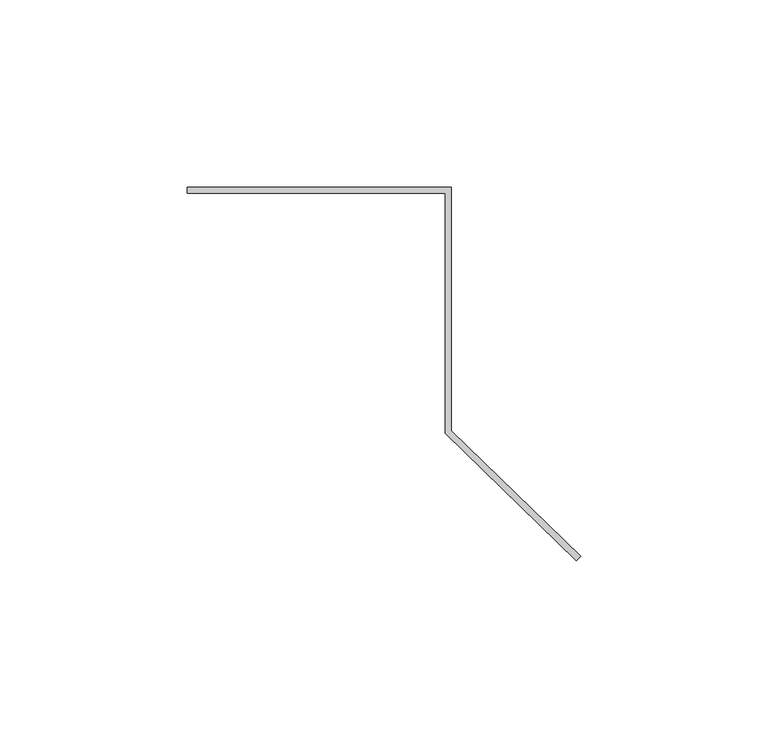
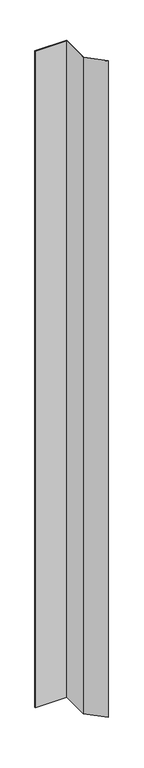
"""IFC4 building model written with IfcOpenShell, lengths in millimetres: proxy geometry, Generic Models 2:Generic Models 2:310765:Generic Models 2:310765 : Generic Models 2:Generic Models 2:310765:61 : Generic Models 2:Generic Models 2:310765:Generic Models 2:310765 : Generic Models 2:Generic Models 2:310765:300385."""

from ifc_helpers import new_model, si_unit, frame, origin, place, context, project, spatial, polyline, outline, extrude, source, transform, mapped, element, save


def generic_models_9b77d285(model_context):
    return source(origin(), model_context, "Body", "SweptSolid", [
        extrude(outline(polyline([(667216.6366489, -568274.0939933), (667286.9617239, -568274.0939933), (667286.9617239, -568339.0177162), (667321.5133229, -568372.5097328), (667320.3906548, -568373.6324009), (667285.3742239, -568339.6898072), (667285.3742239, -568275.6814933), (667216.6366489, -568275.6814933), (667216.6366489, -568274.0939933)])), frame((0.0, 0.0, 4636.9670756), z_axis=(0.0, 0.0, 1.0), x_axis=(1.0, 0.0, 0.0)), (0.0, 0.0, 1.0), 1528.8829244),
    ])


if __name__ == "__main__":
    model = new_model("IFC4")
    model_context = context("Model", 3, world=origin())
    ifc_project = project(units=[si_unit("LENGTHUNIT", "METRE", prefix="MILLI")], contexts=[model_context])
    site = spatial("IfcSite", under=ifc_project)
    building = spatial("IfcBuilding", under=site)
    placement = place(None, origin())
    generic_models_shape = generic_models_9b77d285(model_context)
    element("IfcBuildingElementProxy", 1, Name="Generic Models 2:Generic Models 2:310765:Generic Models 2:310765 : Generic Models 2:Generic Models 2:310765:61 : Generic Models 2:Generic Models 2:310765:Generic Models 2:310765 : Generic Models 2:Generic Models 2:310765:300385", ObjectType="Generic Models 2:Generic Models 2:310765:Generic Models 2:310765 : Generic Models 2:Generic Models 2:310765:61 : Generic Models 2:Generic Models 2:310765:Generic Models 2:310765 : Generic Models 2:Generic Models 2:310765:300385", at=placement, inside=building, context=model_context, shape_type="MappedRepresentation", body=[
        mapped(generic_models_shape, transform((0.0, 0.0, 0.0), x_axis=(1.0, 0.0, 0.0), y_axis=(0.0, 1.0, 0.0), z_axis=(0.0, 0.0, 1.0))),
    ])
    save(model, "model.ifc")

# Revit data of these elements
# Type "Generic Models 2:Generic Models 2:310765:Generic Models 2:310765 : Generic Models 2:Generic Models 2:310765:61 : Generic Models 2:Generic Models 2:310765:Generic Models 2:310765 : Generic Models 2:Generic Models 2:310765:300385"
#   NameOverride = "Generic Models 2:Generic Models 2:310765:Generic Models 2:310765 : Generic Models 2:Generic Models 2:310765:300385"
#   ObjectTypeOverride = "Generic Models 2:310765 : Generic Models 2:Generic Models 2:310765"
#   Reference = "Generic Models 2"
#   Tag = "300385"
# Element 1 (IfcBuildingElementProxy, "Generic Models 2:Generic Models 2:310765:Generic Models 2:310765 : Generic Models 2:Generic Models 2:310765:61 : Generic Models 2:Generic Models 2:310765:Generic Models 2:310765 : Generic Models 2:Generic Models 2:310765:300385")
#   Materials on its faces: "BRAKE METAL CLOSURE TRIM"
# Materials
#   "BRAKE METAL CLOSURE TRIM": class "Unassigned", colour RGB 182 182 182, transparency 0, Cost = 0
